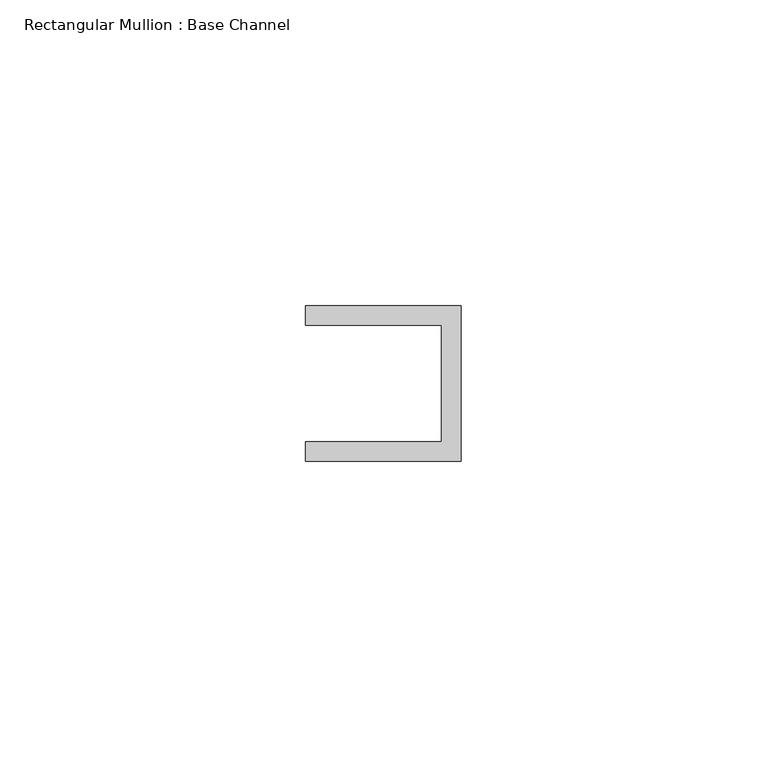
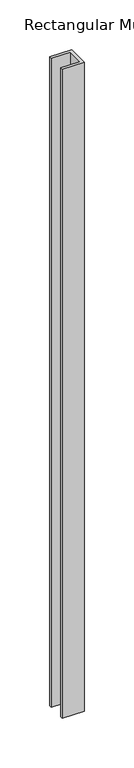
"""IFC4 building model written with IfcOpenShell, lengths in millimetres: member geometry, Rectangular Mullion : Base Channel."""

import ifcopenshell
import ifcopenshell.guid

model = None  # the IFC model being written
_history = None  # IfcOwnerHistory: only IFC2X3 demands one
_inside = {}  # id of a spatial element -> (the spatial element, [elements in it])
_under = {}  # id of a project, library or spatial element -> (it, [spatial elements below it])
_declared = {}  # id of a project -> (the project, [libraries it declares])
_typed = {}  # id of a type object -> (the type object, [elements of that type])
_made_of = {}  # id of a material, layer set ... -> (it, [elements and type objects made of it])


def new_model(schema):
    """Start an empty IFC model of exactly this schema.

    Asked for "IFC4X3", IfcOpenShell would pick the latest addendum, in which some entities
    have other attributes; the version numbers below select the first issue.
    IFC2X3 requires an IfcOwnerHistory on every rooted entity: one is made here for all.
    """
    global model, _history
    if schema == "IFC4X3":
        model = ifcopenshell.file(schema_version=(4, 3, 0, 0))
    else:
        model = ifcopenshell.file(schema=schema)
    _inside.clear()
    _under.clear()
    _declared.clear()
    _typed.clear()
    _made_of.clear()
    _history = None
    if model.schema == "IFC2X3":
        org = make("IfcOrganization", Name="unknown")
        user = make(
            "IfcPersonAndOrganization",
            ThePerson=make("IfcPerson", FamilyName="unknown"),
            TheOrganization=org,
        )
        app = make(
            "IfcApplication",
            ApplicationDeveloper=org,
            Version="unknown",
            ApplicationFullName="unknown",
            ApplicationIdentifier="unknown",
        )
        _history = make(
            "IfcOwnerHistory",
            OwningUser=user,
            OwningApplication=app,
            ChangeAction="ADDED",
            CreationDate=0,
        )
    return model


def make(cls, **values):
    """One entity of the class cls with the attributes given. An attribute that is None is left unset."""
    return model.create_entity(
        cls, **{name: value for name, value in values.items() if value is not None}
    )


def rooted(cls, **values):
    """An entity with a GlobalId (a new one), such as an element, a storey or a relation."""
    return make(cls, GlobalId=ifcopenshell.guid.new(), OwnerHistory=_history, **values)


def si_unit(unit_type, name, prefix=None):
    """IfcSIUnit, for example si_unit("LENGTHUNIT", "METRE", prefix="MILLI")."""
    return make("IfcSIUnit", UnitType=unit_type, Prefix=prefix, Name=name)


def assignment(units):
    """IfcUnitAssignment: the units of a project."""
    return None if units is None else make("IfcUnitAssignment", Units=units)


def point(xyz):
    """IfcCartesianPoint."""
    return None if xyz is None else make("IfcCartesianPoint", Coordinates=xyz)


def direction(xyz):
    """IfcDirection."""
    return None if xyz is None else make("IfcDirection", DirectionRatios=xyz)


def frame(location, z_axis=None, x_axis=None):
    """IfcAxis2Placement3D, a coordinate frame: its origin and axes. An axis left out is left unset."""
    return make(
        "IfcAxis2Placement3D",
        Location=point(location),
        Axis=direction(z_axis),
        RefDirection=direction(x_axis),
    )


def origin():
    """The frame at (0, 0, 0) with its axes left unset."""
    return frame((0.0, 0.0, 0.0))


def place(relative_to, where):
    """IfcLocalPlacement: puts the frame where relative to a parent placement (None: the world)."""
    return make(
        "IfcLocalPlacement", PlacementRelTo=relative_to, RelativePlacement=where
    )


def context(
    kind, dimensions, precision=None, world=None, true_north=None, identifier=None
):
    """IfcGeometricRepresentationContext, for example the 3D "Model" context."""
    return make(
        "IfcGeometricRepresentationContext",
        ContextIdentifier=identifier,
        ContextType=kind,
        CoordinateSpaceDimension=dimensions,
        Precision=precision,
        WorldCoordinateSystem=world,
        TrueNorth=true_north,
    )


def project(units=None, contexts=None):
    """IfcProject with its units and contexts."""
    return rooted(
        "IfcProject",
        Name="project",
        RepresentationContexts=contexts,
        UnitsInContext=assignment(units),
    )


def spatial(cls, under=None, at=None, **own):
    """A site, building, storey or space (cls), placed at a placement, below another one or the project."""
    s = rooted(cls, ObjectPlacement=at, **own)
    if under is not None:
        _under.setdefault(under.id(), (under, []))[1].append(s)
    return s


def polyline(points):
    """IfcPolyline through the points."""
    return make("IfcPolyline", Points=[point(p) for p in points])


def outline(outer, holes=None, kind="AREA"):
    """IfcArbitraryClosedProfileDef: a profile drawn as a closed curve; with holes, ...WithVoids."""
    if holes is None:
        return make("IfcArbitraryClosedProfileDef", ProfileType=kind, OuterCurve=outer)
    return make(
        "IfcArbitraryProfileDefWithVoids",
        ProfileType=kind,
        OuterCurve=outer,
        InnerCurves=holes,
    )


def extrude(swept, where, along, depth):
    """IfcExtrudedAreaSolid: the profile swept, set in the frame where, extruded along a direction by depth."""
    return make(
        "IfcExtrudedAreaSolid",
        SweptArea=swept,
        Position=where,
        ExtrudedDirection=direction(along),
        Depth=depth,
    )


def shape(context_of_items, identifier, shape_type, items):
    """IfcShapeRepresentation: the items that make up one representation, for example the "Body"."""
    return make(
        "IfcShapeRepresentation",
        ContextOfItems=context_of_items,
        RepresentationIdentifier=identifier,
        RepresentationType=shape_type,
        Items=items,
    )


def source(mapping_origin, context_of_items, identifier, shape_type, items):
    """IfcRepresentationMap: a shape defined once, which mapped items show again and again."""
    return make(
        "IfcRepresentationMap",
        MappingOrigin=mapping_origin,
        MappedRepresentation=shape(context_of_items, identifier, shape_type, items),
    )


def transform(
    local_origin,
    x_axis=None,
    y_axis=None,
    z_axis=None,
    scale=None,
    scale2=None,
    scale3=None,
    uniform=True,
):
    """IfcCartesianTransformationOperator3D, or its non-uniform kind. x_axis, y_axis, z_axis: its Axis1, 2, 3."""
    if uniform:
        return make(
            "IfcCartesianTransformationOperator3D",
            Axis1=direction(x_axis),
            Axis2=direction(y_axis),
            LocalOrigin=point(local_origin),
            Scale=scale,
            Axis3=direction(z_axis),
        )
    return make(
        "IfcCartesianTransformationOperator3DnonUniform",
        Axis1=direction(x_axis),
        Axis2=direction(y_axis),
        LocalOrigin=point(local_origin),
        Scale=scale,
        Axis3=direction(z_axis),
        Scale2=scale2,
        Scale3=scale3,
    )


def mapped(mapping_source, mapping_target):
    """IfcMappedItem: shows the shape of a source again, moved by a transform."""
    return make(
        "IfcMappedItem", MappingSource=mapping_source, MappingTarget=mapping_target
    )


def made_of(thing, what):
    """Note that an element or type object is made of a material, layer set ...; save() writes the relation."""
    if what is not None:
        _made_of.setdefault(what.id(), (what, []))[1].append(thing)
    return thing


def element(
    cls,
    number,
    at=None,
    inside=None,
    cuts=None,
    type_object=None,
    material=None,
    context=None,
    identifier="Body",
    shape_type=None,
    held_by="IfcProductDefinitionShape",
    body=None,
    shapes=None,
    **own,
):
    """One element of the class cls, such as IfcWall. Its Tag is "e" and its number.

    at: its placement. inside: the storey or other place that contains it. cuts: it is an
    opening in that element (IfcRelVoidsElement). A single representation is given by context,
    identifier, shape_type and body (its items); several are given by shapes. held_by: the class
    of the entity that holds the representations. save() writes the other relations.
    """
    e = rooted(cls, Tag="e%d" % number, ObjectPlacement=at, **own)
    if body is not None:
        shapes = [shape(context, identifier, shape_type, body)]
    if shapes is not None:
        e.Representation = make(held_by, Representations=shapes)
    if inside is not None:
        _inside.setdefault(inside.id(), (inside, []))[1].append(e)
    if cuts is not None:
        rooted(
            "IfcRelVoidsElement", RelatingBuildingElement=cuts, RelatedOpeningElement=e
        )
    if type_object is not None:
        _typed.setdefault(type_object.id(), (type_object, []))[1].append(e)
    return made_of(e, material)


def aggregate(whole, parts):
    """IfcRelAggregates: a whole, such as a stair, and the parts it consists of."""
    return rooted("IfcRelAggregates", RelatingObject=whole, RelatedObjects=parts)


def save(model, path):
    """Write the relations noted so far, then the file.

    IfcRelAggregates (storeys below a building ...), IfcRelContainedInSpatialStructure (elements
    in a storey), IfcRelDefinesByType, IfcRelAssociatesMaterial and IfcRelDeclares: one each for
    every whole, place, type object, material and project.
    """
    for whole, parts in _under.values():
        aggregate(whole, parts)
    for where, things in _inside.values():
        rooted(
            "IfcRelContainedInSpatialStructure",
            RelatedElements=things,
            RelatingStructure=where,
        )
    for kind, things in _typed.values():
        rooted("IfcRelDefinesByType", RelatedObjects=things, RelatingType=kind)
    for what, things in _made_of.values():
        rooted("IfcRelAssociatesMaterial", RelatedObjects=things, RelatingMaterial=what)
    for by, libraries in _declared.values():
        rooted("IfcRelDeclares", RelatingContext=by, RelatedDefinitions=libraries)
    model.write(path)


def rectangular_mullion_base_channel_d47311eb(model_context):
    return source(origin(), model_context, "Body", "SweptSolid", [
        extrude(outline(polyline([(0.0, -12.7), (-25.4, -12.7), (-25.4, -9.525), (-3.175, -9.525), (-3.175, 9.525), (-25.4, 9.525), (-25.4, 12.7), (0.0, 12.7), (0.0, -12.7)])), frame((0.0, 0.0, -797.4590998), z_axis=(0.0, 0.0, 1.0), x_axis=(1.0, 0.0, 0.0)), (0.0, 0.0, 1.0), 797.4590998),
    ])


if __name__ == "__main__":
    model = new_model("IFC4")
    model_context = context("Model", 3, world=origin())
    ifc_project = project(units=[si_unit("LENGTHUNIT", "METRE", prefix="MILLI")], contexts=[model_context])
    site = spatial("IfcSite", under=ifc_project)
    building = spatial("IfcBuilding", under=site)
    placement = place(None, origin())
    rectangular_mullion_base_channel_shape = rectangular_mullion_base_channel_d47311eb(model_context)
    element("IfcMember", 1, ObjectType="Rectangular Mullion : Base Channel", at=placement, inside=building, context=model_context, shape_type="MappedRepresentation", body=[
        mapped(rectangular_mullion_base_channel_shape, transform((0.0, 0.0, 0.0), x_axis=(1.0, 0.0, 0.0), y_axis=(0.0, 1.0, 0.0), z_axis=(0.0, 0.0, 1.0))),
    ])
    save(model, "model.ifc")

# Revit data of these elements
# Type "Rectangular Mullion : Base Channel"
#   built-in parameter 1007322 = 0.0833333 (stored number, unit not read)
#   built-in parameter 1007321 = 0.0416667 (stored number, unit not read)
#   built-in parameter 1007320 = -0.03125 (stored number, unit not read)
# Element 1 (IfcMember, "Rectangular Mullion : Base Channel")
#   Materials on its faces: "ALUM"
# Materials
#   "ALUM": class "Generic", colour RGB 157 157 157, transparency 0, Cost = 0
